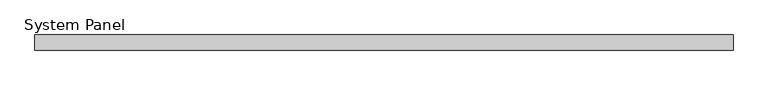
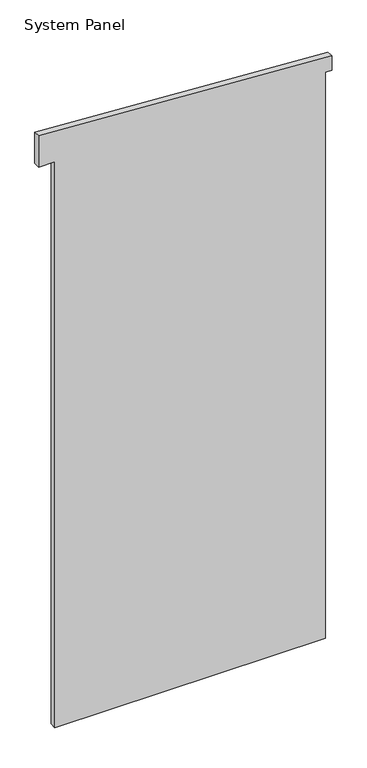
"""IFC4 building model written with IfcOpenShell, lengths in millimetres: plate geometry, System Panel : TEMPERED INSULATED GLAZING (CARDINAL GLASS LoĒ²-240."""

from ifc_helpers import new_model, si_unit, frame, origin, place, context, project, spatial, polyline, outline, extrude, source, transform, mapped, element, save


def system_panel_022879fd(model_context):
    return source(origin(), model_context, "Body", "SweptSolid", [
        extrude(outline(polyline([(0.0, -509.6406773), (0.0, 547.7406773), (2336.3357725, 547.7406773), (2336.3357725, 573.1406773), (2394.2473009, 573.1406773), (2465.8898856, -573.1406773), (2336.3357725, -573.1406773), (2336.3357725, -509.6406773), (0.0, -509.6406773)])), frame((0.0, -31.75, 0.0), z_axis=(0.0, 1.0, 0.0), x_axis=(0.0, 0.0, 1.0)), (0.0, 0.0, 1.0), 25.4),
    ])


if __name__ == "__main__":
    model = new_model("IFC4")
    model_context = context("Model", 3, world=origin())
    ifc_project = project(units=[si_unit("LENGTHUNIT", "METRE", prefix="MILLI")], contexts=[model_context])
    site = spatial("IfcSite", under=ifc_project)
    building = spatial("IfcBuilding", under=site)
    placement = place(None, origin())
    system_panel_shape = system_panel_022879fd(model_context)
    element("IfcPlate", 1, ObjectType="System Panel : TEMPERED INSULATED GLAZING (CARDINAL GLASS LoĒ²-240", at=placement, inside=building, context=model_context, shape_type="MappedRepresentation", body=[
        mapped(system_panel_shape, transform((0.0, 0.0, 0.0), x_axis=(1.0, 0.0, 0.0), y_axis=(0.0, 1.0, 0.0), z_axis=(0.0, 0.0, 1.0))),
    ])
    save(model, "model.ifc")

# Revit data of these elements
# Type "System Panel : TEMPERED INSULATED GLAZING (CARDINAL GLASS LoĒ²-240"
#   Construction Type Id = "opn-s72"
#   Analytic Construction = "Double glazing - 1/4 in thick - low-E/clear (e = 0.1) glass"
#   Visual Light Transmittance = 0.72
#   Solar Heat Gain Coefficient = 0.6
#   Heat Transfer Coefficient (U) = 1.9873 W/(m²·K)
#   Transparency_Hack = 70
# Element 1 (IfcPlate, "System Panel : TEMPERED INSULATED GLAZING (CARDINAL GLASS LoĒ²-240")
#   Materials on its faces: "TEMPERED INSULATED GLAZING (CARDINAL GLASS LoĒ²-240\nOR EQUIVALENT)"
# Materials
#   "TEMPERED INSULATED GLAZING (CARDINAL GLASS LoĒ²-240\nOR EQUIVALENT)": class "Glass", colour RGB 196 205 210, transparency 0.85, Description = "Soda Lime Glass", Cost = 0
